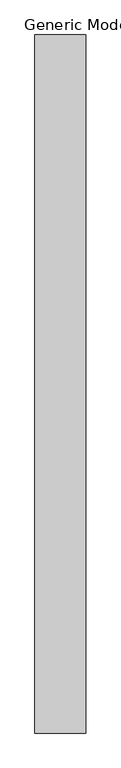
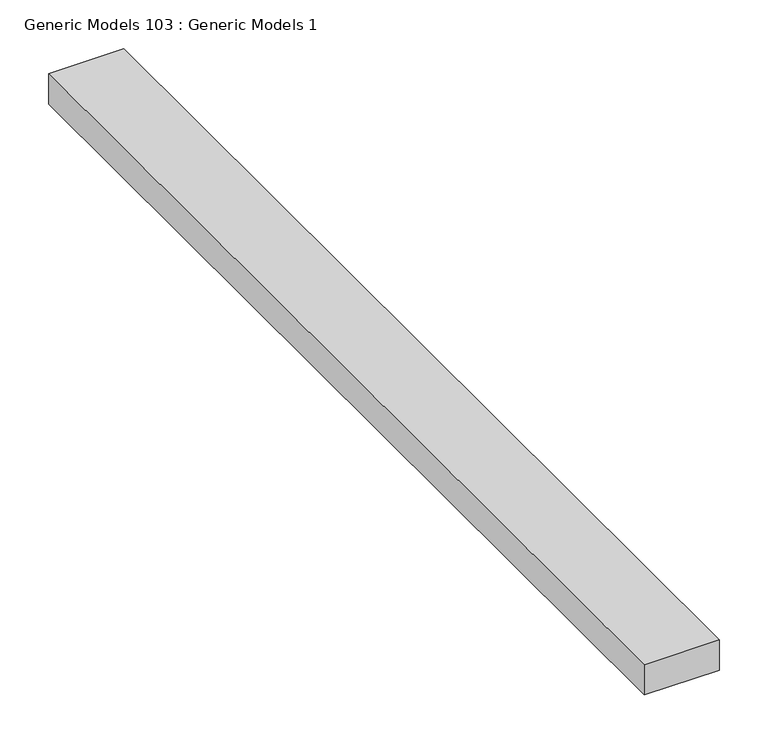
"""IFC4 building model written with IfcOpenShell, lengths in millimetres: proxy geometry, Generic Models 103 : Generic Models 1."""

import ifcopenshell
import ifcopenshell.guid

model = None  # the IFC model being written
_history = None  # IfcOwnerHistory: only IFC2X3 demands one
_inside = {}  # id of a spatial element -> (the spatial element, [elements in it])
_under = {}  # id of a project, library or spatial element -> (it, [spatial elements below it])
_declared = {}  # id of a project -> (the project, [libraries it declares])
_typed = {}  # id of a type object -> (the type object, [elements of that type])
_made_of = {}  # id of a material, layer set ... -> (it, [elements and type objects made of it])


def new_model(schema):
    """Start an empty IFC model of exactly this schema.

    Asked for "IFC4X3", IfcOpenShell would pick the latest addendum, in which some entities
    have other attributes; the version numbers below select the first issue.
    IFC2X3 requires an IfcOwnerHistory on every rooted entity: one is made here for all.
    """
    global model, _history
    if schema == "IFC4X3":
        model = ifcopenshell.file(schema_version=(4, 3, 0, 0))
    else:
        model = ifcopenshell.file(schema=schema)
    _inside.clear()
    _under.clear()
    _declared.clear()
    _typed.clear()
    _made_of.clear()
    _history = None
    if model.schema == "IFC2X3":
        org = make("IfcOrganization", Name="unknown")
        user = make(
            "IfcPersonAndOrganization",
            ThePerson=make("IfcPerson", FamilyName="unknown"),
            TheOrganization=org,
        )
        app = make(
            "IfcApplication",
            ApplicationDeveloper=org,
            Version="unknown",
            ApplicationFullName="unknown",
            ApplicationIdentifier="unknown",
        )
        _history = make(
            "IfcOwnerHistory",
            OwningUser=user,
            OwningApplication=app,
            ChangeAction="ADDED",
            CreationDate=0,
        )
    return model


def make(cls, **values):
    """One entity of the class cls with the attributes given. An attribute that is None is left unset."""
    return model.create_entity(
        cls, **{name: value for name, value in values.items() if value is not None}
    )


def rooted(cls, **values):
    """An entity with a GlobalId (a new one), such as an element, a storey or a relation."""
    return make(cls, GlobalId=ifcopenshell.guid.new(), OwnerHistory=_history, **values)


def si_unit(unit_type, name, prefix=None):
    """IfcSIUnit, for example si_unit("LENGTHUNIT", "METRE", prefix="MILLI")."""
    return make("IfcSIUnit", UnitType=unit_type, Prefix=prefix, Name=name)


def assignment(units):
    """IfcUnitAssignment: the units of a project."""
    return None if units is None else make("IfcUnitAssignment", Units=units)


def point(xyz):
    """IfcCartesianPoint."""
    return None if xyz is None else make("IfcCartesianPoint", Coordinates=xyz)


def direction(xyz):
    """IfcDirection."""
    return None if xyz is None else make("IfcDirection", DirectionRatios=xyz)


def frame(location, z_axis=None, x_axis=None):
    """IfcAxis2Placement3D, a coordinate frame: its origin and axes. An axis left out is left unset."""
    return make(
        "IfcAxis2Placement3D",
        Location=point(location),
        Axis=direction(z_axis),
        RefDirection=direction(x_axis),
    )


def origin():
    """The frame at (0, 0, 0) with its axes left unset."""
    return frame((0.0, 0.0, 0.0))


def place(relative_to, where):
    """IfcLocalPlacement: puts the frame where relative to a parent placement (None: the world)."""
    return make(
        "IfcLocalPlacement", PlacementRelTo=relative_to, RelativePlacement=where
    )


def context(
    kind, dimensions, precision=None, world=None, true_north=None, identifier=None
):
    """IfcGeometricRepresentationContext, for example the 3D "Model" context."""
    return make(
        "IfcGeometricRepresentationContext",
        ContextIdentifier=identifier,
        ContextType=kind,
        CoordinateSpaceDimension=dimensions,
        Precision=precision,
        WorldCoordinateSystem=world,
        TrueNorth=true_north,
    )


def project(units=None, contexts=None):
    """IfcProject with its units and contexts."""
    return rooted(
        "IfcProject",
        Name="project",
        RepresentationContexts=contexts,
        UnitsInContext=assignment(units),
    )


def spatial(cls, under=None, at=None, **own):
    """A site, building, storey or space (cls), placed at a placement, below another one or the project."""
    s = rooted(cls, ObjectPlacement=at, **own)
    if under is not None:
        _under.setdefault(under.id(), (under, []))[1].append(s)
    return s


def polyline(points):
    """IfcPolyline through the points."""
    return make("IfcPolyline", Points=[point(p) for p in points])


def outline(outer, holes=None, kind="AREA"):
    """IfcArbitraryClosedProfileDef: a profile drawn as a closed curve; with holes, ...WithVoids."""
    if holes is None:
        return make("IfcArbitraryClosedProfileDef", ProfileType=kind, OuterCurve=outer)
    return make(
        "IfcArbitraryProfileDefWithVoids",
        ProfileType=kind,
        OuterCurve=outer,
        InnerCurves=holes,
    )


def extrude(swept, where, along, depth):
    """IfcExtrudedAreaSolid: the profile swept, set in the frame where, extruded along a direction by depth."""
    return make(
        "IfcExtrudedAreaSolid",
        SweptArea=swept,
        Position=where,
        ExtrudedDirection=direction(along),
        Depth=depth,
    )


def shape(context_of_items, identifier, shape_type, items):
    """IfcShapeRepresentation: the items that make up one representation, for example the "Body"."""
    return make(
        "IfcShapeRepresentation",
        ContextOfItems=context_of_items,
        RepresentationIdentifier=identifier,
        RepresentationType=shape_type,
        Items=items,
    )


def source(mapping_origin, context_of_items, identifier, shape_type, items):
    """IfcRepresentationMap: a shape defined once, which mapped items show again and again."""
    return make(
        "IfcRepresentationMap",
        MappingOrigin=mapping_origin,
        MappedRepresentation=shape(context_of_items, identifier, shape_type, items),
    )


def transform(
    local_origin,
    x_axis=None,
    y_axis=None,
    z_axis=None,
    scale=None,
    scale2=None,
    scale3=None,
    uniform=True,
):
    """IfcCartesianTransformationOperator3D, or its non-uniform kind. x_axis, y_axis, z_axis: its Axis1, 2, 3."""
    if uniform:
        return make(
            "IfcCartesianTransformationOperator3D",
            Axis1=direction(x_axis),
            Axis2=direction(y_axis),
            LocalOrigin=point(local_origin),
            Scale=scale,
            Axis3=direction(z_axis),
        )
    return make(
        "IfcCartesianTransformationOperator3DnonUniform",
        Axis1=direction(x_axis),
        Axis2=direction(y_axis),
        LocalOrigin=point(local_origin),
        Scale=scale,
        Axis3=direction(z_axis),
        Scale2=scale2,
        Scale3=scale3,
    )


def mapped(mapping_source, mapping_target):
    """IfcMappedItem: shows the shape of a source again, moved by a transform."""
    return make(
        "IfcMappedItem", MappingSource=mapping_source, MappingTarget=mapping_target
    )


def made_of(thing, what):
    """Note that an element or type object is made of a material, layer set ...; save() writes the relation."""
    if what is not None:
        _made_of.setdefault(what.id(), (what, []))[1].append(thing)
    return thing


def element(
    cls,
    number,
    at=None,
    inside=None,
    cuts=None,
    type_object=None,
    material=None,
    context=None,
    identifier="Body",
    shape_type=None,
    held_by="IfcProductDefinitionShape",
    body=None,
    shapes=None,
    **own,
):
    """One element of the class cls, such as IfcWall. Its Tag is "e" and its number.

    at: its placement. inside: the storey or other place that contains it. cuts: it is an
    opening in that element (IfcRelVoidsElement). A single representation is given by context,
    identifier, shape_type and body (its items); several are given by shapes. held_by: the class
    of the entity that holds the representations. save() writes the other relations.
    """
    e = rooted(cls, Tag="e%d" % number, ObjectPlacement=at, **own)
    if body is not None:
        shapes = [shape(context, identifier, shape_type, body)]
    if shapes is not None:
        e.Representation = make(held_by, Representations=shapes)
    if inside is not None:
        _inside.setdefault(inside.id(), (inside, []))[1].append(e)
    if cuts is not None:
        rooted(
            "IfcRelVoidsElement", RelatingBuildingElement=cuts, RelatedOpeningElement=e
        )
    if type_object is not None:
        _typed.setdefault(type_object.id(), (type_object, []))[1].append(e)
    return made_of(e, material)


def aggregate(whole, parts):
    """IfcRelAggregates: a whole, such as a stair, and the parts it consists of."""
    return rooted("IfcRelAggregates", RelatingObject=whole, RelatedObjects=parts)


def save(model, path):
    """Write the relations noted so far, then the file.

    IfcRelAggregates (storeys below a building ...), IfcRelContainedInSpatialStructure (elements
    in a storey), IfcRelDefinesByType, IfcRelAssociatesMaterial and IfcRelDeclares: one each for
    every whole, place, type object, material and project.
    """
    for whole, parts in _under.values():
        aggregate(whole, parts)
    for where, things in _inside.values():
        rooted(
            "IfcRelContainedInSpatialStructure",
            RelatedElements=things,
            RelatingStructure=where,
        )
    for kind, things in _typed.values():
        rooted("IfcRelDefinesByType", RelatedObjects=things, RelatingType=kind)
    for what, things in _made_of.values():
        rooted("IfcRelAssociatesMaterial", RelatedObjects=things, RelatingMaterial=what)
    for by, libraries in _declared.values():
        rooted("IfcRelDeclares", RelatingContext=by, RelatedDefinitions=libraries)
    model.write(path)


def generic_models_103_generic_models_1_250a6a11(model_context):
    return source(origin(), model_context, "Body", "SweptSolid", [
        extrude(outline(polyline([(49784.0, 0.0), (49695.1, 0.0), (49695.1, 1219.2), (49784.0, 1219.2), (49784.0, 0.0)])), frame((0.0, 0.0, 5264.15), z_axis=(0.0, 0.0, 1.0), x_axis=(1.0, 0.0, 0.0)), (0.0, 0.0, 1.0), 38.1),
    ])


if __name__ == "__main__":
    model = new_model("IFC4")
    model_context = context("Model", 3, world=origin())
    ifc_project = project(units=[si_unit("LENGTHUNIT", "METRE", prefix="MILLI")], contexts=[model_context])
    site = spatial("IfcSite", under=ifc_project)
    building = spatial("IfcBuilding", under=site)
    placement = place(None, origin())
    generic_models_103_generic_models_1_shape = generic_models_103_generic_models_1_250a6a11(model_context)
    element("IfcBuildingElementProxy", 1, Name="Generic Models 103 : Generic Models 1", ObjectType="Generic Models 103 : Generic Models 1", at=placement, inside=building, context=model_context, shape_type="MappedRepresentation", body=[
        mapped(generic_models_103_generic_models_1_shape, transform((0.0, 0.0, 0.0), x_axis=(1.0, 0.0, 0.0), y_axis=(0.0, 1.0, 0.0), z_axis=(0.0, 0.0, 1.0))),
    ])
    save(model, "model.ifc")

# Revit data of these elements
# Element 1 (IfcBuildingElementProxy, "Generic Models 103 : Generic Models 1")
#   Materials on its faces: "2X WOOD HEADER ATTACHED TO STEEL PURLIN"
# Materials
#   "2X WOOD HEADER ATTACHED TO STEEL PURLIN": class "Wood", colour RGB 234 198 147, transparency 0, Description = "Pinus Echinata", Cost = 0
